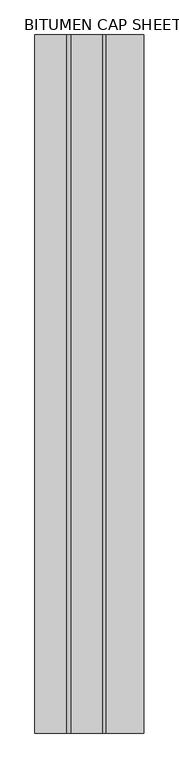
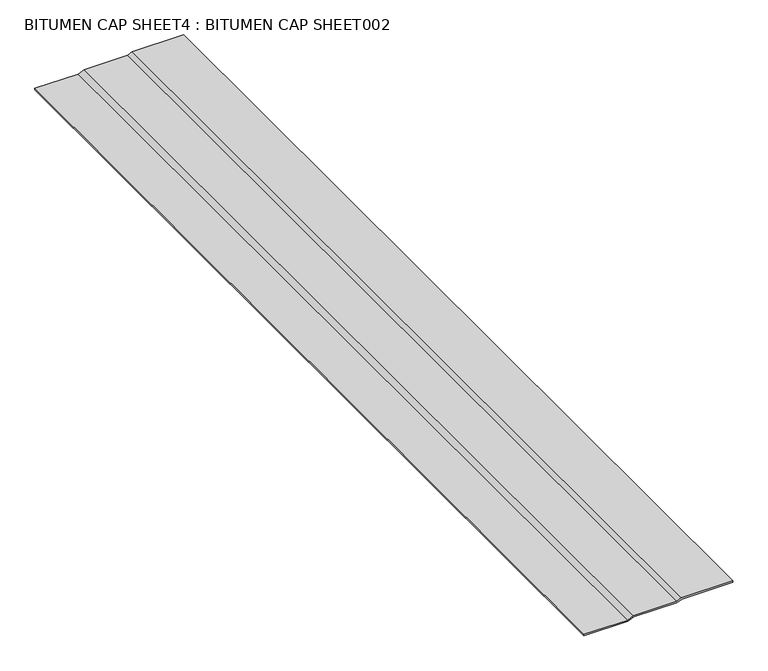
"""IFC4 building model written with IfcOpenShell, lengths in millimetres: proxy geometry, BITUMEN CAP SHEET4 : BITUMEN CAP SHEET002."""

from ifc_helpers import new_model, si_unit, frame, origin, place, context, project, spatial, polyline, outline, extrude, source, transform, mapped, element, save


def bitumen_cap_sheet4_bitumen_cap_sheet002_cc5fe4d3(model_context):
    return source(origin(), model_context, "Body", "SweptSolid", [
        extrude(outline(polyline([(40259.2002678, -4699.8063764), (40259.2002678, -4607.6417148), (40264.4862773, -4595.1768962), (40264.4862773, -4504.46274), (40268.8188423, -4494.7463535), (40268.8188423, -4387.5351424), (40271.9940719, -4387.5351424), (40271.9940719, -4495.421639), (40267.6612773, -4505.1385405), (40267.6612773, -4595.8222961), (40262.3752678, -4608.2871148), (40262.3752678, -4699.8063764), (40259.2002678, -4699.8063764)])), frame((0.0, -1052.8906574, 0.0), z_axis=(0.0, 1.0, 0.0), x_axis=(0.0, 0.0, 1.0)), (0.0, 0.0, 1.0), 2000.25),
    ])


if __name__ == "__main__":
    model = new_model("IFC4")
    model_context = context("Model", 3, world=origin())
    ifc_project = project(units=[si_unit("LENGTHUNIT", "METRE", prefix="MILLI")], contexts=[model_context])
    site = spatial("IfcSite", under=ifc_project)
    building = spatial("IfcBuilding", under=site)
    placement = place(None, origin())
    bitumen_cap_sheet4_bitumen_cap_sheet002_shape = bitumen_cap_sheet4_bitumen_cap_sheet002_cc5fe4d3(model_context)
    element("IfcBuildingElementProxy", 1, Name="BITUMEN CAP SHEET4 : BITUMEN CAP SHEET002", ObjectType="BITUMEN CAP SHEET4 : BITUMEN CAP SHEET002", at=placement, inside=building, context=model_context, shape_type="MappedRepresentation", body=[
        mapped(bitumen_cap_sheet4_bitumen_cap_sheet002_shape, transform((0.0, 0.0, 0.0), x_axis=(1.0, 0.0, 0.0), y_axis=(0.0, 1.0, 0.0), z_axis=(0.0, 0.0, 1.0))),
    ])
    save(model, "model.ifc")

# Revit data of these elements
# Type "BITUMEN CAP SHEET4 : BITUMEN CAP SHEET002"
#   NameOverride = "BITUMEN CAP SHEET002"
# Element 1 (IfcBuildingElementProxy, "BITUMEN CAP SHEET4 : BITUMEN CAP SHEET002")
#   Materials on its faces: "MODIFIED BITUMEN GRANULE SURFACED CAP SHEET"
# Materials
#   "MODIFIED BITUMEN GRANULE SURFACED CAP SHEET": class "Unassigned", colour RGB 85 85 127, transparency 0
